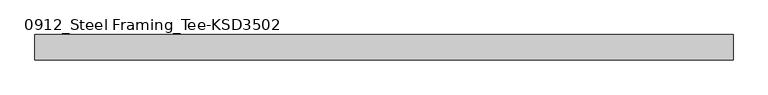
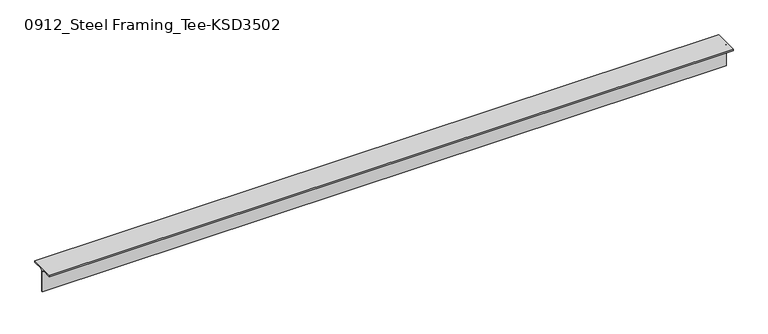
"""IFC4 building model written with IfcOpenShell, lengths in millimetres: member geometry, 0912_Steel Framing_Tee-KSD3502 : H_SB_ASB_CT-150x150x6.5x9."""

from ifc_helpers import new_model, si_unit, point, frame, frame_2d, origin, place, context, project, spatial, polyline, circle_curve, trimmed, segment, composite_curve, outline, extrude, source, transform, mapped, element, save


def member_0912_steel_framing_tee_ksd3502_cd65d3bd(model_context):
    return source(origin(), model_context, "Body", "SweptSolid", [
        extrude(outline(composite_curve([segment(polyline([(-75.0, 75.0), (75.0, 75.0), (75.0, 66.0), (16.25, 66.0)]), True, "CONTINUOUS"), segment(trimmed(circle_curve(frame_2d((16.25, 53.0)), 13.0), [point((16.25, 66.0))], [point((3.25, 53.0))], True, "CARTESIAN"), True, "CONTINUOUS"), segment(polyline([(3.25, 53.0), (3.25, -75.0), (-3.25, -75.0), (-3.25, 53.0)]), True, "CONTINUOUS"), segment(trimmed(circle_curve(frame_2d((-16.25, 53.0)), 13.0), [point((-3.25, 53.0))], [point((-16.25, 66.0))], True, "CARTESIAN"), True, "CONTINUOUS"), segment(polyline([(-16.25, 66.0), (-75.0, 66.0), (-75.0, 75.0)]), True, "CONTINUOUS")], self_intersect=False)), frame((-2093.85, 0.0, 0.0), z_axis=(1.0, 0.0, 0.0), x_axis=(0.0, 1.0, 0.0)), (0.0, 0.0, 1.0), 4122.7),
    ])


if __name__ == "__main__":
    model = new_model("IFC4")
    model_context = context("Model", 3, world=origin())
    ifc_project = project(units=[si_unit("LENGTHUNIT", "METRE", prefix="MILLI")], contexts=[model_context])
    site = spatial("IfcSite", under=ifc_project)
    building = spatial("IfcBuilding", under=site)
    placement = place(None, origin())
    member_0912_steel_framing_tee_ksd3502_shape = member_0912_steel_framing_tee_ksd3502_cd65d3bd(model_context)
    element("IfcMember", 1, ObjectType="0912_Steel Framing_Tee-KSD3502 : H_SB_ASB_CT-150x150x6.5x9", at=placement, inside=building, context=model_context, shape_type="MappedRepresentation", body=[
        mapped(member_0912_steel_framing_tee_ksd3502_shape, transform((0.0, 0.0, 0.0), x_axis=(1.0, 0.0, 0.0), y_axis=(0.0, 1.0, 0.0), z_axis=(0.0, 0.0, 1.0))),
    ])
    save(model, "model.ifc")

# Revit data of these elements
# Type "0912_Steel Framing_Tee-KSD3502 : H_SB_ASB_CT-150x150x6.5x9"
#   H_WM Code_1 = "S01AA003-00001 | Main Steel Structure Fabrication Work | Shelter/Building | Light Steel - Standard (30KG/M>Weight) | Material: (   )"
#   H_WM Code_2 = "S03AA029-00001 | Main Steel Structure Erection Work | Shelter/Building | Light Steel (30KG/M>Weight) | Material: (   )"
#   H_WM Code_3 = "S01AA010-00001 | Main Steel Structure Fabrication Work | Shelter/Building | Steel Painting/Coating | for Non-Fireproofed Steel Surface, Surface Preparation, Primer, Second & Final Coat | Material: (   )"
#   H_Q'ty Cal Type Tag = "SB-Q2"
#   Width = 15.0 cm
#   Web Thickness = 0.65 cm
#   Web Fillet = 1.3 cm
#   Section Area = 23.39 cm²
#   Perimeter = 0.60 m²/m
#   Nominal Weight = 18.40 kgf/m
#   Height = 15.0 cm
#   Flange Thickness = 0.9 cm
#   Centroid Vertical = 7.5 cm
#   Centroid Horizontal = 7.5 cm
#   Length [instance default] = 1.5000 m
#   Structural Material [instance default] = Steel, 45-345
#   Warping Constant = (empty or 0)
#   Torsional Moment of Inertia = 0
#   Section Name Key = ""
#   Plastic Modulus weak axis = 0
#   Plastic Modulus strong axis = 0
#   Moment of Inertia weak axis = 0
#   Moment of Inertia strong axis = 0
#   Elastic Modulus weak axis = 0
#   Elastic Modulus strong axis = 0
#   Bolt Spacing = 0
#   Assembly Code = ""
# Element 1 (IfcMember, "0912_Steel Framing_Tee-KSD3502 : H_SB_ASB_CT-150x150x6.5x9")
#   Structural Material = none
# Materials
#   "Steel, 45-345": class "Metal", colour RGB 189 187 185, transparency 0, Description = "Steel 345 MPa", Cost = 0
